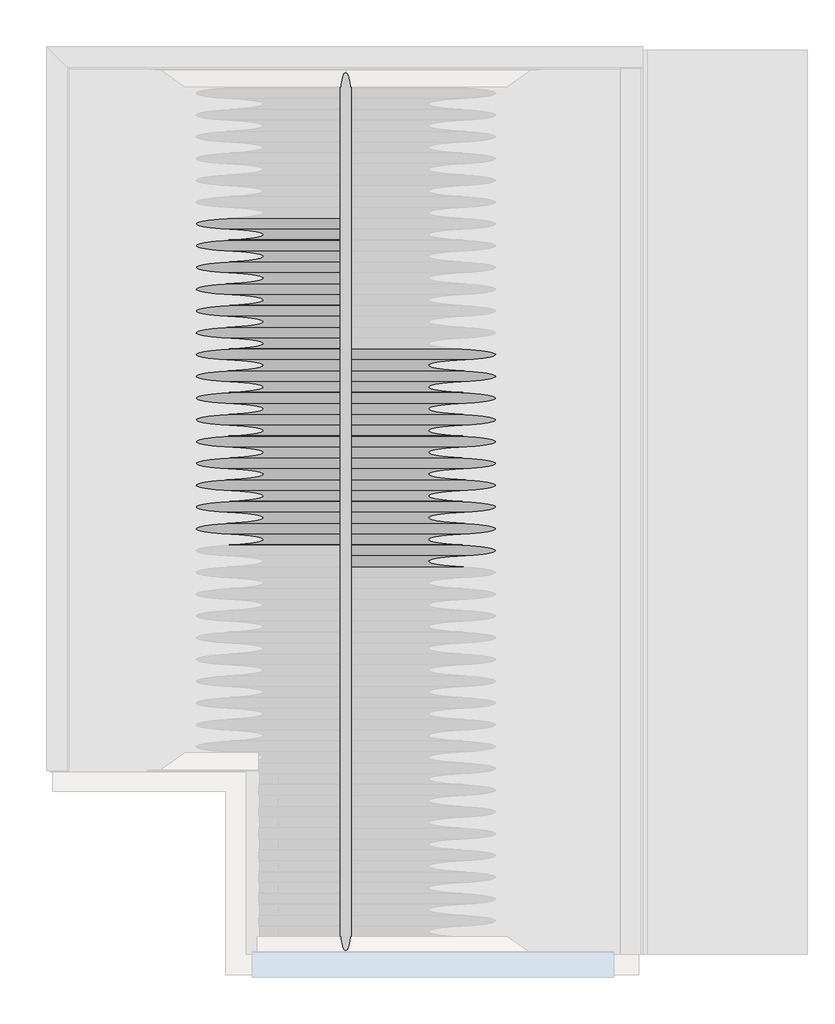
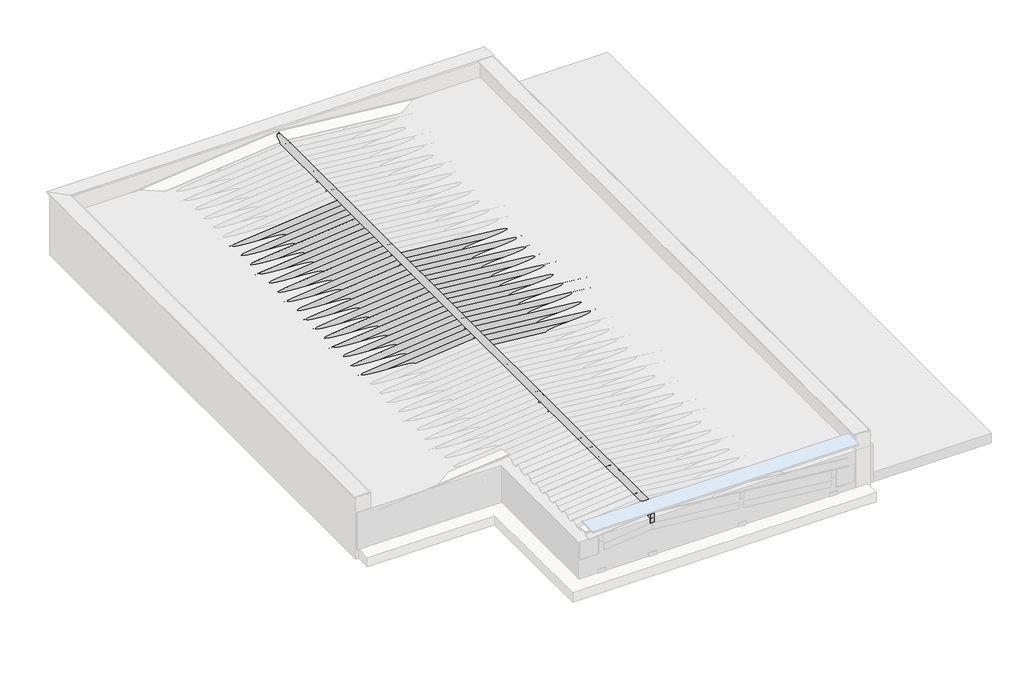
# One storey, part 3 of 4: 34 beams, 7 columns.
"""IFC4 building model written with IfcOpenShell, lengths in millimetres."""

import ifcopenshell
import ifcopenshell.guid

model = None  # the IFC model being written
_history = None  # IfcOwnerHistory: only IFC2X3 demands one
_inside = {}  # id of a spatial element -> (the spatial element, [elements in it])
_under = {}  # id of a project, library or spatial element -> (it, [spatial elements below it])
_declared = {}  # id of a project -> (the project, [libraries it declares])
_typed = {}  # id of a type object -> (the type object, [elements of that type])
_made_of = {}  # id of a material, layer set ... -> (it, [elements and type objects made of it])


def new_model(schema):
    """Start an empty IFC model of exactly this schema.

    Asked for "IFC4X3", IfcOpenShell would pick the latest addendum, in which some entities
    have other attributes; the version numbers below select the first issue.
    IFC2X3 requires an IfcOwnerHistory on every rooted entity: one is made here for all.
    """
    global model, _history
    if schema == "IFC4X3":
        model = ifcopenshell.file(schema_version=(4, 3, 0, 0))
    else:
        model = ifcopenshell.file(schema=schema)
    _inside.clear()
    _under.clear()
    _declared.clear()
    _typed.clear()
    _made_of.clear()
    _history = None
    if model.schema == "IFC2X3":
        org = make("IfcOrganization", Name="unknown")
        user = make(
            "IfcPersonAndOrganization",
            ThePerson=make("IfcPerson", FamilyName="unknown"),
            TheOrganization=org,
        )
        app = make(
            "IfcApplication",
            ApplicationDeveloper=org,
            Version="unknown",
            ApplicationFullName="unknown",
            ApplicationIdentifier="unknown",
        )
        _history = make(
            "IfcOwnerHistory",
            OwningUser=user,
            OwningApplication=app,
            ChangeAction="ADDED",
            CreationDate=0,
        )
    return model


def make(cls, **values):
    """One entity of the class cls with the attributes given. An attribute that is None is left unset."""
    return model.create_entity(
        cls, **{name: value for name, value in values.items() if value is not None}
    )


def rooted(cls, **values):
    """An entity with a GlobalId (a new one), such as an element, a storey or a relation."""
    return make(cls, GlobalId=ifcopenshell.guid.new(), OwnerHistory=_history, **values)


def si_unit(unit_type, name, prefix=None):
    """IfcSIUnit, for example si_unit("LENGTHUNIT", "METRE", prefix="MILLI")."""
    return make("IfcSIUnit", UnitType=unit_type, Prefix=prefix, Name=name)


def assignment(units):
    """IfcUnitAssignment: the units of a project."""
    return None if units is None else make("IfcUnitAssignment", Units=units)


def point(xyz):
    """IfcCartesianPoint."""
    return None if xyz is None else make("IfcCartesianPoint", Coordinates=xyz)


def direction(xyz):
    """IfcDirection."""
    return None if xyz is None else make("IfcDirection", DirectionRatios=xyz)


def frame(location, z_axis=None, x_axis=None):
    """IfcAxis2Placement3D, a coordinate frame: its origin and axes. An axis left out is left unset."""
    return make(
        "IfcAxis2Placement3D",
        Location=point(location),
        Axis=direction(z_axis),
        RefDirection=direction(x_axis),
    )


def frame_2d(location, x_axis=None):
    """IfcAxis2Placement2D, a coordinate frame in the plane: its origin and x axis."""
    return make(
        "IfcAxis2Placement2D", Location=point(location), RefDirection=direction(x_axis)
    )


def origin():
    """The frame at (0, 0, 0) with its axes left unset."""
    return frame((0.0, 0.0, 0.0))


def place(relative_to, where):
    """IfcLocalPlacement: puts the frame where relative to a parent placement (None: the world)."""
    return make(
        "IfcLocalPlacement", PlacementRelTo=relative_to, RelativePlacement=where
    )


def context(
    kind, dimensions, precision=None, world=None, true_north=None, identifier=None
):
    """IfcGeometricRepresentationContext, for example the 3D "Model" context."""
    return make(
        "IfcGeometricRepresentationContext",
        ContextIdentifier=identifier,
        ContextType=kind,
        CoordinateSpaceDimension=dimensions,
        Precision=precision,
        WorldCoordinateSystem=world,
        TrueNorth=true_north,
    )


def project(units=None, contexts=None):
    """IfcProject with its units and contexts."""
    return rooted(
        "IfcProject",
        Name="project",
        RepresentationContexts=contexts,
        UnitsInContext=assignment(units),
    )


def spatial(cls, under=None, at=None, **own):
    """A site, building, storey or space (cls), placed at a placement, below another one or the project."""
    s = rooted(cls, ObjectPlacement=at, **own)
    if under is not None:
        _under.setdefault(under.id(), (under, []))[1].append(s)
    return s


def polyline(points):
    """IfcPolyline through the points."""
    return make("IfcPolyline", Points=[point(p) for p in points])


def circle_curve(where, radius):
    """IfcCircle in the frame where."""
    return make("IfcCircle", Position=where, Radius=radius)


def trimmed(basis, trim1, trim2, sense, master):
    """IfcTrimmedCurve: the piece of a basis curve between two trims."""
    return make(
        "IfcTrimmedCurve",
        BasisCurve=basis,
        Trim1=trim1,
        Trim2=trim2,
        SenseAgreement=sense,
        MasterRepresentation=master,
    )


def segment(curve, same_sense, transition):
    """IfcCompositeCurveSegment."""
    return make(
        "IfcCompositeCurveSegment",
        Transition=transition,
        SameSense=same_sense,
        ParentCurve=curve,
    )


def composite_curve(segments, self_intersect=None):
    """IfcCompositeCurve: segments joined end to end."""
    return make("IfcCompositeCurve", Segments=segments, SelfIntersect=self_intersect)


def outline(outer, holes=None, kind="AREA"):
    """IfcArbitraryClosedProfileDef: a profile drawn as a closed curve; with holes, ...WithVoids."""
    if holes is None:
        return make("IfcArbitraryClosedProfileDef", ProfileType=kind, OuterCurve=outer)
    return make(
        "IfcArbitraryProfileDefWithVoids",
        ProfileType=kind,
        OuterCurve=outer,
        InnerCurves=holes,
    )


def extrude(swept, where, along, depth):
    """IfcExtrudedAreaSolid: the profile swept, set in the frame where, extruded along a direction by depth."""
    return make(
        "IfcExtrudedAreaSolid",
        SweptArea=swept,
        Position=where,
        ExtrudedDirection=direction(along),
        Depth=depth,
    )


def shape(context_of_items, identifier, shape_type, items):
    """IfcShapeRepresentation: the items that make up one representation, for example the "Body"."""
    return make(
        "IfcShapeRepresentation",
        ContextOfItems=context_of_items,
        RepresentationIdentifier=identifier,
        RepresentationType=shape_type,
        Items=items,
    )


def source(mapping_origin, context_of_items, identifier, shape_type, items):
    """IfcRepresentationMap: a shape defined once, which mapped items show again and again."""
    return make(
        "IfcRepresentationMap",
        MappingOrigin=mapping_origin,
        MappedRepresentation=shape(context_of_items, identifier, shape_type, items),
    )


def transform(
    local_origin,
    x_axis=None,
    y_axis=None,
    z_axis=None,
    scale=None,
    scale2=None,
    scale3=None,
    uniform=True,
):
    """IfcCartesianTransformationOperator3D, or its non-uniform kind. x_axis, y_axis, z_axis: its Axis1, 2, 3."""
    if uniform:
        return make(
            "IfcCartesianTransformationOperator3D",
            Axis1=direction(x_axis),
            Axis2=direction(y_axis),
            LocalOrigin=point(local_origin),
            Scale=scale,
            Axis3=direction(z_axis),
        )
    return make(
        "IfcCartesianTransformationOperator3DnonUniform",
        Axis1=direction(x_axis),
        Axis2=direction(y_axis),
        LocalOrigin=point(local_origin),
        Scale=scale,
        Axis3=direction(z_axis),
        Scale2=scale2,
        Scale3=scale3,
    )


def mapped(mapping_source, mapping_target):
    """IfcMappedItem: shows the shape of a source again, moved by a transform."""
    return make(
        "IfcMappedItem", MappingSource=mapping_source, MappingTarget=mapping_target
    )


def made_of(thing, what):
    """Note that an element or type object is made of a material, layer set ...; save() writes the relation."""
    if what is not None:
        _made_of.setdefault(what.id(), (what, []))[1].append(thing)
    return thing


def element(
    cls,
    number,
    at=None,
    inside=None,
    cuts=None,
    type_object=None,
    material=None,
    context=None,
    identifier="Body",
    shape_type=None,
    held_by="IfcProductDefinitionShape",
    body=None,
    shapes=None,
    **own,
):
    """One element of the class cls, such as IfcWall. Its Tag is "e" and its number.

    at: its placement. inside: the storey or other place that contains it. cuts: it is an
    opening in that element (IfcRelVoidsElement). A single representation is given by context,
    identifier, shape_type and body (its items); several are given by shapes. held_by: the class
    of the entity that holds the representations. save() writes the other relations.
    """
    e = rooted(cls, Tag="e%d" % number, ObjectPlacement=at, **own)
    if body is not None:
        shapes = [shape(context, identifier, shape_type, body)]
    if shapes is not None:
        e.Representation = make(held_by, Representations=shapes)
    if inside is not None:
        _inside.setdefault(inside.id(), (inside, []))[1].append(e)
    if cuts is not None:
        rooted(
            "IfcRelVoidsElement", RelatingBuildingElement=cuts, RelatedOpeningElement=e
        )
    if type_object is not None:
        _typed.setdefault(type_object.id(), (type_object, []))[1].append(e)
    return made_of(e, material)


def aggregate(whole, parts):
    """IfcRelAggregates: a whole, such as a stair, and the parts it consists of."""
    return rooted("IfcRelAggregates", RelatingObject=whole, RelatedObjects=parts)


def save(model, path):
    """Write the relations noted so far, then the file.

    IfcRelAggregates (storeys below a building ...), IfcRelContainedInSpatialStructure (elements
    in a storey), IfcRelDefinesByType, IfcRelAssociatesMaterial and IfcRelDeclares: one each for
    every whole, place, type object, material and project.
    """
    for whole, parts in _under.values():
        aggregate(whole, parts)
    for where, things in _inside.values():
        rooted(
            "IfcRelContainedInSpatialStructure",
            RelatedElements=things,
            RelatingStructure=where,
        )
    for kind, things in _typed.values():
        rooted("IfcRelDefinesByType", RelatedObjects=things, RelatingType=kind)
    for what, things in _made_of.values():
        rooted("IfcRelAssociatesMaterial", RelatedObjects=things, RelatingMaterial=what)
    for by, libraries in _declared.values():
        rooted("IfcRelDeclares", RelatingContext=by, RelatedDefinitions=libraries)
    model.write(path)


def cumeeira_telha_ondulada_fibrocimento_c9eafb3e(model_context):
    return source(origin(), model_context, "Body", "SweptSolid", [
        extrude(outline(composite_curve([segment(polyline([(58.3970135, 42.4437972), (53.9055884, 40.2467307)]), True, "CONTINUOUS"), segment(trimmed(circle_curve(frame_2d((-1.6029865, 13.0936483)), 61.7939461), [point((53.9055884, 40.2467307))], [point((-57.1115615, 40.2467307))], True, "CARTESIAN"), True, "CONTINUOUS"), segment(polyline([(-57.1115615, 40.2467307), (-61.6029865, 42.4437972)]), True, "CONTINUOUS"), segment(trimmed(circle_curve(frame_2d((-1.6029865, 13.0936483)), 66.7939461), [point((-61.6029865, 42.4437972))], [point((58.3970135, 42.4437972))], False, "CARTESIAN"), True, "CONTINUOUS")], self_intersect=False)), frame((-4969.5, 0.0, 0.0), z_axis=(1.0, 0.0, 0.0), x_axis=(0.0, 1.0, 0.0)), (0.0, 0.0, 1.0), 9939.0),
    ])


def viga_cumeeira_6x16cm_10b61863(model_context):
    return source(origin(), model_context, "Body", "SweptSolid", [
        extrude(outline(polyline([(4969.4999994, 30.0), (4969.4999994, -30.0), (-4969.4999994, -30.0), (-4969.4999994, 30.0), (4969.4999994, 30.0)])), frame((0.0, 0.0, -80.0), z_axis=(0.0, 0.0, 1.0), x_axis=(1.0, 0.0, 0.0)), (0.0, 0.0, 1.0), 160.0),
    ])


def column_7d6827b5(model_context):
    return source(origin(), model_context, "Body", "SweptSolid", [
        extrude(outline(polyline([(30.0, 80.0), (30.0, -80.0), (-30.0, -80.0), (-30.0, 80.0), (30.0, 80.0)])), frame((0.0, 0.0, 4460.0), z_axis=(0.0, 0.0, 1.0), x_axis=(1.0, 0.0, 0.0)), (0.0, 0.0, 1.0), 466.0),
    ])


def column_c7348c99(model_context):
    return source(origin(), model_context, "Body", "SweptSolid", [
        extrude(outline(polyline([(30.0, 80.0), (30.0, -80.0), (-30.0, -80.0), (-30.0, 80.0), (30.0, 80.0)])), frame((0.0, 0.0, 4460.0), z_axis=(0.0, 0.0, 1.0), x_axis=(1.0, 0.0, 0.0)), (0.0, 0.0, 1.0), 372.8),
    ])


def column_6cc9e01b(model_context):
    return source(origin(), model_context, "Body", "SweptSolid", [
        extrude(outline(polyline([(30.0, 80.0), (30.0, -80.0), (-30.0, -80.0), (-30.0, 80.0), (30.0, 80.0)])), frame((0.0, 0.0, 4460.0), z_axis=(0.0, 0.0, 1.0), x_axis=(1.0, 0.0, 0.0)), (0.0, 0.0, 1.0), 233.0),
    ])


model = new_model("IFC4")

# Units and contexts
model_context = context("Model", 3, world=origin())
ifc_project = project(units=[si_unit("LENGTHUNIT", "METRE", prefix="MILLI")], contexts=[model_context])

# Site, building, storey
site = spatial("IfcSite", under=ifc_project)
building = spatial("IfcBuilding", under=site)
storey = spatial("IfcBuildingStorey", under=building, Name="COB. SALA ESTAR", Elevation=4400.0)

# Beams
placement = place(None, origin())
element("IfcBeam", 1, ObjectType="Madeira de lei : Berço 6x12cm", at=placement, inside=storey, context=model_context, shape_type="SweptSolid", body=[
    extrude(outline(polyline([(-3400.8557491, 2180.4300147), (-3280.8557491, 2180.4300147), (-3280.8557491, 180.4300153), (-3400.8557491, 180.4300153), (-3400.8557491, 2180.4300147)])), frame((0.0, 0.0, 4400.0), z_axis=(0.0, 0.0, 1.0), x_axis=(1.0, 0.0, 0.0)), (0.0, 0.0, 1.0), 60.0),
])
element("IfcBeam", 2, ObjectType="Madeira de lei : Berço 6x12cm", at=placement, inside=storey, context=model_context, shape_type="SweptSolid", body=[
    extrude(outline(polyline([(-3400.8557491, 4180.4300153), (-3280.8557491, 4180.4300153), (-3280.8557491, 2180.4300159), (-3400.8557491, 2180.4300159), (-3400.8557491, 4180.4300153)])), frame((0.0, 0.0, 4400.0), z_axis=(0.0, 0.0, 1.0), x_axis=(1.0, 0.0, 0.0)), (0.0, 0.0, 1.0), 60.0),
])
element("IfcBeam", 3, ObjectType="Madeira de lei : Berço 6x12cm", at=placement, inside=storey, context=model_context, shape_type="SweptSolid", body=[
    extrude(outline(polyline([(-2032.3324227, 2180.4300147), (-1912.3324227, 2180.4300147), (-1912.3324227, 180.4300153), (-2032.3324227, 180.4300153), (-2032.3324227, 2180.4300147)])), frame((0.0, 0.0, 4400.0), z_axis=(0.0, 0.0, 1.0), x_axis=(1.0, 0.0, 0.0)), (0.0, 0.0, 1.0), 60.0),
])
element("IfcBeam", 4, ObjectType="Madeira de lei : Berço 6x12cm", at=placement, inside=storey, context=model_context, shape_type="SweptSolid", body=[
    extrude(outline(polyline([(-634.0324227, 2180.4300147), (-514.0324227, 2180.4300147), (-514.0324227, 180.4300153), (-634.0324227, 180.4300153), (-634.0324227, 2180.4300147)])), frame((0.0, 0.0, 4400.0), z_axis=(0.0, 0.0, 1.0), x_axis=(1.0, 0.0, 0.0)), (0.0, 0.0, 1.0), 60.0),
])
element("IfcBeam", 5, ObjectType="Madeira de lei : Berço 6x12cm", at=placement, inside=storey, context=model_context, shape_type="SweptSolid", body=[
    extrude(outline(polyline([(-6167.5301913, 4180.4300153), (-6047.5301913, 4180.4300153), (-6047.5301913, 2180.4300159), (-6167.5301913, 2180.4300159), (-6167.5301913, 4180.4300153)])), frame((0.0, 0.0, 4400.0), z_axis=(0.0, 0.0, 1.0), x_axis=(1.0, 0.0, 0.0)), (0.0, 0.0, 1.0), 60.0),
])
element("IfcBeam", 6, ObjectType="Madeira de lei : Berço 6x12cm", at=placement, inside=storey, context=model_context, shape_type="SweptSolid", body=[
    extrude(outline(polyline([(-4769.2301913, 2180.4300147), (-4649.2301913, 2180.4300147), (-4649.2301913, 180.4300153), (-4769.2301913, 180.4300153), (-4769.2301913, 2180.4300147)])), frame((0.0, 0.0, 4400.0), z_axis=(0.0, 0.0, 1.0), x_axis=(1.0, 0.0, 0.0)), (0.0, 0.0, 1.0), 60.0),
])
element("IfcBeam", 7, ObjectType="Madeira de lei : Berço 6x12cm", at=placement, inside=storey, context=model_context, shape_type="SweptSolid", body=[
    extrude(outline(polyline([(-4769.2301913, 4180.4300153), (-4649.2301913, 4180.4300153), (-4649.2301913, 2180.4300159), (-4769.2301913, 2180.4300159), (-4769.2301913, 4180.4300153)])), frame((0.0, 0.0, 4400.0), z_axis=(0.0, 0.0, 1.0), x_axis=(1.0, 0.0, 0.0)), (0.0, 0.0, 1.0), 60.0),
])
cumeeira_telha_ondulada_fibrocimento_shape = cumeeira_telha_ondulada_fibrocimento_c9eafb3e(model_context)
element("IfcBeam", 8, ObjectType="Cumeeira Telha Ondulada : Fibrocimento", at=placement, inside=storey, context=model_context, shape_type="MappedRepresentation", body=[
    mapped(cumeeira_telha_ondulada_fibrocimento_shape, transform((-3340.8557491, 623.9300153, 5123.1251229), x_axis=(0.0, -1.0, 0.0), y_axis=(1.0, 0.0, 0.0), z_axis=(0.0, 0.0, 1.0))),
])
element("IfcBeam", 9, ObjectType="Telha Ondulada : Fibrocimento", at=placement, inside=storey, context=model_context, shape_type="SweptSolid", body=[
    extrude(outline(composite_curve([segment(trimmed(circle_curve(frame_2d((-58.7002978, -53.2060538)), 66.7939461), [point((-29.3501489, 6.7939462))], [point((-29.3501489, -113.2060538))], False, "CARTESIAN"), True, "CONTINUOUS"), segment(polyline([(-29.3501489, -113.2060538), (-31.5472154, -108.7146288)]), True, "CONTINUOUS"), segment(trimmed(circle_curve(frame_2d((-58.7002978, -53.2060538)), 61.7939461), [point((-31.5472154, -108.7146288))], [point((-31.5472154, 2.3025211))], True, "CARTESIAN"), True, "CONTINUOUS"), segment(trimmed(circle_curve(frame_2d((0.0, 66.7939462)), 71.7939461), [point((-31.5472154, 2.3025211))], [point((-31.5472154, 131.2853712))], False, "CARTESIAN"), True, "CONTINUOUS"), segment(polyline([(-31.5472154, 131.2853712), (-29.3501489, 126.7939462)]), True, "CONTINUOUS"), segment(trimmed(circle_curve(frame_2d((0.0, 66.7939462)), 66.7939461), [point((-29.3501489, 126.7939462))], [point((-29.3501489, 6.7939462))], True, "CARTESIAN"), True, "CONTINUOUS")], self_intersect=False)), frame((-6307.6707245, 377.826948, 4862.7215886), z_axis=(0.9950371902099892, 0.0, 0.09950371902099972), x_axis=(-0.09950371902099972, 0.0, 0.9950371902099892)), (0.0, 0.0, 1.0), 2972.5075682),
])
element("IfcBeam", 10, ObjectType="Telha Ondulada : Fibrocimento", at=placement, inside=storey, context=model_context, shape_type="SweptSolid", body=[
    extrude(outline(composite_curve([segment(trimmed(circle_curve(frame_2d((-58.7002978, -53.2060538)), 66.7939461), [point((-29.3501489, 6.7939462))], [point((-29.3501489, -113.2060538))], False, "CARTESIAN"), True, "CONTINUOUS"), segment(polyline([(-29.3501489, -113.2060538), (-31.5472154, -108.7146288)]), True, "CONTINUOUS"), segment(trimmed(circle_curve(frame_2d((-58.7002978, -53.2060538)), 61.7939461), [point((-31.5472154, -108.7146288))], [point((-31.5472154, 2.3025211))], True, "CARTESIAN"), True, "CONTINUOUS"), segment(trimmed(circle_curve(frame_2d((0.0, 66.7939462)), 71.7939461), [point((-31.5472154, 2.3025211))], [point((-31.5472154, 131.2853712))], False, "CARTESIAN"), True, "CONTINUOUS"), segment(polyline([(-31.5472154, 131.2853712), (-29.3501489, 126.7939462)]), True, "CONTINUOUS"), segment(trimmed(circle_curve(frame_2d((0.0, 66.7939462)), 66.7939461), [point((-29.3501489, 126.7939462))], [point((-29.3501489, 6.7939462))], True, "CARTESIAN"), True, "CONTINUOUS")], self_intersect=False)), frame((-6307.6707245, 622.326948, 4862.7215886), z_axis=(0.9950371902099892, 0.0, 0.09950371902099972), x_axis=(-0.09950371902099972, 0.0, 0.9950371902099892)), (0.0, 0.0, 1.0), 2972.5075682),
])
element("IfcBeam", 11, ObjectType="Telha Ondulada : Fibrocimento", at=placement, inside=storey, context=model_context, shape_type="SweptSolid", body=[
    extrude(outline(composite_curve([segment(trimmed(circle_curve(frame_2d((-58.7002978, -53.2060538)), 66.7939461), [point((-29.3501489, 6.7939462))], [point((-29.3501489, -113.2060538))], False, "CARTESIAN"), True, "CONTINUOUS"), segment(polyline([(-29.3501489, -113.2060538), (-31.5472154, -108.7146288)]), True, "CONTINUOUS"), segment(trimmed(circle_curve(frame_2d((-58.7002978, -53.2060538)), 61.7939461), [point((-31.5472154, -108.7146288))], [point((-31.5472154, 2.3025211))], True, "CARTESIAN"), True, "CONTINUOUS"), segment(trimmed(circle_curve(frame_2d((0.0, 66.7939462)), 71.7939461), [point((-31.5472154, 2.3025211))], [point((-31.5472154, 131.2853712))], False, "CARTESIAN"), True, "CONTINUOUS"), segment(polyline([(-31.5472154, 131.2853712), (-29.3501489, 126.7939462)]), True, "CONTINUOUS"), segment(trimmed(circle_curve(frame_2d((0.0, 66.7939462)), 66.7939461), [point((-29.3501489, 126.7939462))], [point((-29.3501489, 6.7939462))], True, "CARTESIAN"), True, "CONTINUOUS")], self_intersect=False)), frame((-6307.6707245, 866.826948, 4862.7215886), z_axis=(0.9950371902099892, 0.0, 0.09950371902099968), x_axis=(-0.09950371902099968, 0.0, 0.9950371902099892)), (0.0, 0.0, 1.0), 2972.5075682),
])
element("IfcBeam", 12, ObjectType="Telha Ondulada : Fibrocimento", at=placement, inside=storey, context=model_context, shape_type="SweptSolid", body=[
    extrude(outline(composite_curve([segment(trimmed(circle_curve(frame_2d((-58.7002978, -53.2060538)), 66.7939461), [point((-29.3501489, 6.7939462))], [point((-29.3501489, -113.2060538))], False, "CARTESIAN"), True, "CONTINUOUS"), segment(polyline([(-29.3501489, -113.2060538), (-31.5472154, -108.7146288)]), True, "CONTINUOUS"), segment(trimmed(circle_curve(frame_2d((-58.7002978, -53.2060538)), 61.7939461), [point((-31.5472154, -108.7146288))], [point((-31.5472154, 2.3025211))], True, "CARTESIAN"), True, "CONTINUOUS"), segment(trimmed(circle_curve(frame_2d((0.0, 66.7939462)), 71.7939461), [point((-31.5472154, 2.3025211))], [point((-31.5472154, 131.2853712))], False, "CARTESIAN"), True, "CONTINUOUS"), segment(polyline([(-31.5472154, 131.2853712), (-29.3501489, 126.7939462)]), True, "CONTINUOUS"), segment(trimmed(circle_curve(frame_2d((0.0, 66.7939462)), 66.7939461), [point((-29.3501489, 126.7939462))], [point((-29.3501489, 6.7939462))], True, "CARTESIAN"), True, "CONTINUOUS")], self_intersect=False)), frame((-6307.6707245, 1111.326948, 4862.7215886), z_axis=(0.9950371902099892, 0.0, 0.09950371902099972), x_axis=(-0.09950371902099972, 0.0, 0.9950371902099892)), (0.0, 0.0, 1.0), 2972.5075682),
])
element("IfcBeam", 13, ObjectType="Telha Ondulada : Fibrocimento", at=placement, inside=storey, context=model_context, shape_type="SweptSolid", body=[
    extrude(outline(composite_curve([segment(trimmed(circle_curve(frame_2d((-58.7002978, -53.2060538)), 66.7939461), [point((-29.3501489, 6.7939462))], [point((-29.3501489, -113.2060538))], False, "CARTESIAN"), True, "CONTINUOUS"), segment(polyline([(-29.3501489, -113.2060538), (-31.5472154, -108.7146288)]), True, "CONTINUOUS"), segment(trimmed(circle_curve(frame_2d((-58.7002978, -53.2060538)), 61.7939461), [point((-31.5472154, -108.7146288))], [point((-31.5472154, 2.3025211))], True, "CARTESIAN"), True, "CONTINUOUS"), segment(trimmed(circle_curve(frame_2d((0.0, 66.7939462)), 71.7939461), [point((-31.5472154, 2.3025211))], [point((-31.5472154, 131.2853712))], False, "CARTESIAN"), True, "CONTINUOUS"), segment(polyline([(-31.5472154, 131.2853712), (-29.3501489, 126.7939462)]), True, "CONTINUOUS"), segment(trimmed(circle_curve(frame_2d((0.0, 66.7939462)), 66.7939461), [point((-29.3501489, 126.7939462))], [point((-29.3501489, 6.7939462))], True, "CARTESIAN"), True, "CONTINUOUS")], self_intersect=False)), frame((-6307.6707245, 1355.826948, 4862.7215886), z_axis=(0.9950371902099892, 0.0, 0.09950371902099969), x_axis=(-0.09950371902099969, 0.0, 0.9950371902099892)), (0.0, 0.0, 1.0), 2972.5075682),
])
element("IfcBeam", 14, ObjectType="Telha Ondulada : Fibrocimento", at=placement, inside=storey, context=model_context, shape_type="SweptSolid", body=[
    extrude(outline(composite_curve([segment(trimmed(circle_curve(frame_2d((-58.7002978, -53.2060538)), 66.7939461), [point((-29.3501489, 6.7939462))], [point((-29.3501489, -113.2060538))], False, "CARTESIAN"), True, "CONTINUOUS"), segment(polyline([(-29.3501489, -113.2060538), (-31.5472154, -108.7146288)]), True, "CONTINUOUS"), segment(trimmed(circle_curve(frame_2d((-58.7002978, -53.2060538)), 61.7939461), [point((-31.5472154, -108.7146288))], [point((-31.5472154, 2.3025211))], True, "CARTESIAN"), True, "CONTINUOUS"), segment(trimmed(circle_curve(frame_2d((0.0, 66.7939462)), 71.7939461), [point((-31.5472154, 2.3025211))], [point((-31.5472154, 131.2853712))], False, "CARTESIAN"), True, "CONTINUOUS"), segment(polyline([(-31.5472154, 131.2853712), (-29.3501489, 126.7939462)]), True, "CONTINUOUS"), segment(trimmed(circle_curve(frame_2d((0.0, 66.7939462)), 66.7939461), [point((-29.3501489, 126.7939462))], [point((-29.3501489, 6.7939462))], True, "CARTESIAN"), True, "CONTINUOUS")], self_intersect=False)), frame((-6307.6707245, 1600.326948, 4862.7215886), z_axis=(0.9950371902099892, 0.0, 0.09950371902099972), x_axis=(-0.09950371902099972, 0.0, 0.9950371902099892)), (0.0, 0.0, 1.0), 2972.5075682),
])
element("IfcBeam", 15, ObjectType="Telha Ondulada : Fibrocimento", at=placement, inside=storey, context=model_context, shape_type="SweptSolid", body=[
    extrude(outline(composite_curve([segment(trimmed(circle_curve(frame_2d((-58.7002978, -53.2060538)), 66.7939461), [point((-29.3501489, 6.7939462))], [point((-29.3501489, -113.2060538))], False, "CARTESIAN"), True, "CONTINUOUS"), segment(polyline([(-29.3501489, -113.2060538), (-31.5472154, -108.7146288)]), True, "CONTINUOUS"), segment(trimmed(circle_curve(frame_2d((-58.7002978, -53.2060538)), 61.7939461), [point((-31.5472154, -108.7146288))], [point((-31.5472154, 2.3025211))], True, "CARTESIAN"), True, "CONTINUOUS"), segment(trimmed(circle_curve(frame_2d((0.0, 66.7939462)), 71.7939461), [point((-31.5472154, 2.3025211))], [point((-31.5472154, 131.2853712))], False, "CARTESIAN"), True, "CONTINUOUS"), segment(polyline([(-31.5472154, 131.2853712), (-29.3501489, 126.7939462)]), True, "CONTINUOUS"), segment(trimmed(circle_curve(frame_2d((0.0, 66.7939462)), 66.7939461), [point((-29.3501489, 126.7939462))], [point((-29.3501489, 6.7939462))], True, "CARTESIAN"), True, "CONTINUOUS")], self_intersect=False)), frame((-6307.6707245, 1844.826948, 4862.7215886), z_axis=(0.9950371902099892, 0.0, 0.09950371902099972), x_axis=(-0.09950371902099972, 0.0, 0.9950371902099892)), (0.0, 0.0, 1.0), 2972.5075682),
])
element("IfcBeam", 16, ObjectType="Telha Ondulada : Fibrocimento", at=placement, inside=storey, context=model_context, shape_type="SweptSolid", body=[
    extrude(outline(composite_curve([segment(trimmed(circle_curve(frame_2d((-58.7002978, -53.2060538)), 66.7939461), [point((-29.3501489, 6.7939462))], [point((-29.3501489, -113.2060538))], False, "CARTESIAN"), True, "CONTINUOUS"), segment(polyline([(-29.3501489, -113.2060538), (-31.5472154, -108.7146288)]), True, "CONTINUOUS"), segment(trimmed(circle_curve(frame_2d((-58.7002978, -53.2060538)), 61.7939461), [point((-31.5472154, -108.7146288))], [point((-31.5472154, 2.3025211))], True, "CARTESIAN"), True, "CONTINUOUS"), segment(trimmed(circle_curve(frame_2d((0.0, 66.7939462)), 71.7939461), [point((-31.5472154, 2.3025211))], [point((-31.5472154, 131.2853712))], False, "CARTESIAN"), True, "CONTINUOUS"), segment(polyline([(-31.5472154, 131.2853712), (-29.3501489, 126.7939462)]), True, "CONTINUOUS"), segment(trimmed(circle_curve(frame_2d((0.0, 66.7939462)), 66.7939461), [point((-29.3501489, 126.7939462))], [point((-29.3501489, 6.7939462))], True, "CARTESIAN"), True, "CONTINUOUS")], self_intersect=False)), frame((-6307.6707245, 2089.326948, 4862.7215886), z_axis=(0.9950371902099892, 0.0, 0.09950371902099954), x_axis=(-0.09950371902099954, 0.0, 0.9950371902099892)), (0.0, 0.0, 1.0), 2972.5075682),
])
element("IfcBeam", 17, ObjectType="Telha Ondulada : Fibrocimento", at=placement, inside=storey, context=model_context, shape_type="SweptSolid", body=[
    extrude(outline(composite_curve([segment(trimmed(circle_curve(frame_2d((-58.7002978, -53.2060538)), 66.7939461), [point((-29.3501489, 6.7939462))], [point((-29.3501489, -113.2060538))], False, "CARTESIAN"), True, "CONTINUOUS"), segment(polyline([(-29.3501489, -113.2060538), (-31.5472154, -108.7146288)]), True, "CONTINUOUS"), segment(trimmed(circle_curve(frame_2d((-58.7002978, -53.2060538)), 61.7939461), [point((-31.5472154, -108.7146288))], [point((-31.5472154, 2.3025211))], True, "CARTESIAN"), True, "CONTINUOUS"), segment(trimmed(circle_curve(frame_2d((0.0, 66.7939462)), 71.7939461), [point((-31.5472154, 2.3025211))], [point((-31.5472154, 131.2853712))], False, "CARTESIAN"), True, "CONTINUOUS"), segment(polyline([(-31.5472154, 131.2853712), (-29.3501489, 126.7939462)]), True, "CONTINUOUS"), segment(trimmed(circle_curve(frame_2d((0.0, 66.7939462)), 66.7939461), [point((-29.3501489, 126.7939462))], [point((-29.3501489, 6.7939462))], True, "CARTESIAN"), True, "CONTINUOUS")], self_intersect=False)), frame((-6307.6707245, 2333.826948, 4862.7215886), z_axis=(0.9950371902099892, 0.0, 0.09950371902099972), x_axis=(-0.09950371902099972, 0.0, 0.9950371902099892)), (0.0, 0.0, 1.0), 2972.5075682),
])
element("IfcBeam", 18, ObjectType="Telha Ondulada : Fibrocimento", at=placement, inside=storey, context=model_context, shape_type="SweptSolid", body=[
    extrude(outline(composite_curve([segment(trimmed(circle_curve(frame_2d((-58.7002978, -53.2060538)), 66.7939461), [point((-29.3501489, 6.7939462))], [point((-29.3501489, -113.2060538))], False, "CARTESIAN"), True, "CONTINUOUS"), segment(polyline([(-29.3501489, -113.2060538), (-31.5472154, -108.7146288)]), True, "CONTINUOUS"), segment(trimmed(circle_curve(frame_2d((-58.7002978, -53.2060538)), 61.7939461), [point((-31.5472154, -108.7146288))], [point((-31.5472154, 2.3025211))], True, "CARTESIAN"), True, "CONTINUOUS"), segment(trimmed(circle_curve(frame_2d((0.0, 66.7939462)), 71.7939461), [point((-31.5472154, 2.3025211))], [point((-31.5472154, 131.2853712))], False, "CARTESIAN"), True, "CONTINUOUS"), segment(polyline([(-31.5472154, 131.2853712), (-29.3501489, 126.7939462)]), True, "CONTINUOUS"), segment(trimmed(circle_curve(frame_2d((0.0, 66.7939462)), 66.7939461), [point((-29.3501489, 126.7939462))], [point((-29.3501489, 6.7939462))], True, "CARTESIAN"), True, "CONTINUOUS")], self_intersect=False)), frame((-6307.6707245, 2578.326948, 4862.7215886), z_axis=(0.9950371902099892, 0.0, 0.09950371902099969), x_axis=(-0.09950371902099969, 0.0, 0.9950371902099892)), (0.0, 0.0, 1.0), 2972.5075682),
])
element("IfcBeam", 19, ObjectType="Telha Ondulada : Fibrocimento", at=placement, inside=storey, context=model_context, shape_type="SweptSolid", body=[
    extrude(outline(composite_curve([segment(trimmed(circle_curve(frame_2d((-58.7002978, -53.2060538)), 66.7939461), [point((-29.3501489, 6.7939462))], [point((-29.3501489, -113.2060538))], False, "CARTESIAN"), True, "CONTINUOUS"), segment(polyline([(-29.3501489, -113.2060538), (-31.5472154, -108.7146288)]), True, "CONTINUOUS"), segment(trimmed(circle_curve(frame_2d((-58.7002978, -53.2060538)), 61.7939461), [point((-31.5472154, -108.7146288))], [point((-31.5472154, 2.3025211))], True, "CARTESIAN"), True, "CONTINUOUS"), segment(trimmed(circle_curve(frame_2d((0.0, 66.7939462)), 71.7939461), [point((-31.5472154, 2.3025211))], [point((-31.5472154, 131.2853712))], False, "CARTESIAN"), True, "CONTINUOUS"), segment(polyline([(-31.5472154, 131.2853712), (-29.3501489, 126.7939462)]), True, "CONTINUOUS"), segment(trimmed(circle_curve(frame_2d((0.0, 66.7939462)), 66.7939461), [point((-29.3501489, 126.7939462))], [point((-29.3501489, 6.7939462))], True, "CARTESIAN"), True, "CONTINUOUS")], self_intersect=False)), frame((-6307.6707245, 2822.826948, 4862.7215886), z_axis=(0.9950371902099892, 0.0, 0.09950371902099972), x_axis=(-0.09950371902099972, 0.0, 0.9950371902099892)), (0.0, 0.0, 1.0), 2972.5075682),
])
element("IfcBeam", 20, ObjectType="Telha Ondulada : Fibrocimento", at=placement, inside=storey, context=model_context, shape_type="SweptSolid", body=[
    extrude(outline(composite_curve([segment(trimmed(circle_curve(frame_2d((-58.7002978, -53.2060538)), 66.7939461), [point((-29.3501489, 6.7939462))], [point((-29.3501489, -113.2060538))], False, "CARTESIAN"), True, "CONTINUOUS"), segment(polyline([(-29.3501489, -113.2060538), (-31.5472154, -108.7146288)]), True, "CONTINUOUS"), segment(trimmed(circle_curve(frame_2d((-58.7002978, -53.2060538)), 61.7939461), [point((-31.5472154, -108.7146288))], [point((-31.5472154, 2.3025211))], True, "CARTESIAN"), True, "CONTINUOUS"), segment(trimmed(circle_curve(frame_2d((0.0, 66.7939462)), 71.7939461), [point((-31.5472154, 2.3025211))], [point((-31.5472154, 131.2853712))], False, "CARTESIAN"), True, "CONTINUOUS"), segment(polyline([(-31.5472154, 131.2853712), (-29.3501489, 126.7939462)]), True, "CONTINUOUS"), segment(trimmed(circle_curve(frame_2d((0.0, 66.7939462)), 66.7939461), [point((-29.3501489, 126.7939462))], [point((-29.3501489, 6.7939462))], True, "CARTESIAN"), True, "CONTINUOUS")], self_intersect=False)), frame((-6307.6707245, 3067.326948, 4862.7215886), z_axis=(0.9950371902099892, 0.0, 0.09950371902099972), x_axis=(-0.09950371902099972, 0.0, 0.9950371902099892)), (0.0, 0.0, 1.0), 2972.5075682),
])
element("IfcBeam", 21, ObjectType="Telha Ondulada : Fibrocimento", at=placement, inside=storey, context=model_context, shape_type="SweptSolid", body=[
    extrude(outline(composite_curve([segment(trimmed(circle_curve(frame_2d((-58.7002978, -53.2060538)), 66.7939461), [point((-29.3501489, 6.7939462))], [point((-29.3501489, -113.2060538))], False, "CARTESIAN"), True, "CONTINUOUS"), segment(polyline([(-29.3501489, -113.2060538), (-31.5472154, -108.7146288)]), True, "CONTINUOUS"), segment(trimmed(circle_curve(frame_2d((-58.7002978, -53.2060538)), 61.7939461), [point((-31.5472154, -108.7146288))], [point((-31.5472154, 2.3025211))], True, "CARTESIAN"), True, "CONTINUOUS"), segment(trimmed(circle_curve(frame_2d((0.0, 66.7939462)), 71.7939461), [point((-31.5472154, 2.3025211))], [point((-31.5472154, 131.2853712))], False, "CARTESIAN"), True, "CONTINUOUS"), segment(polyline([(-31.5472154, 131.2853712), (-29.3501489, 126.7939462)]), True, "CONTINUOUS"), segment(trimmed(circle_curve(frame_2d((0.0, 66.7939462)), 66.7939461), [point((-29.3501489, 126.7939462))], [point((-29.3501489, 6.7939462))], True, "CARTESIAN"), True, "CONTINUOUS")], self_intersect=False)), frame((-6307.6707245, 3311.826948, 4862.7215886), z_axis=(0.9950371902099892, 0.0, 0.09950371902099954), x_axis=(-0.09950371902099954, 0.0, 0.9950371902099892)), (0.0, 0.0, 1.0), 2972.5075682),
])
element("IfcBeam", 22, ObjectType="Telha Ondulada : Fibrocimento", at=placement, inside=storey, context=model_context, shape_type="SweptSolid", body=[
    extrude(outline(composite_curve([segment(trimmed(circle_curve(frame_2d((-58.7002978, -53.2060538)), 66.7939461), [point((-29.3501489, 6.7939462))], [point((-29.3501489, -113.2060538))], False, "CARTESIAN"), True, "CONTINUOUS"), segment(polyline([(-29.3501489, -113.2060538), (-31.5472154, -108.7146288)]), True, "CONTINUOUS"), segment(trimmed(circle_curve(frame_2d((-58.7002978, -53.2060538)), 61.7939461), [point((-31.5472154, -108.7146288))], [point((-31.5472154, 2.3025211))], True, "CARTESIAN"), True, "CONTINUOUS"), segment(trimmed(circle_curve(frame_2d((0.0, 66.7939462)), 71.7939461), [point((-31.5472154, 2.3025211))], [point((-31.5472154, 131.2853712))], False, "CARTESIAN"), True, "CONTINUOUS"), segment(polyline([(-31.5472154, 131.2853712), (-29.3501489, 126.7939462)]), True, "CONTINUOUS"), segment(trimmed(circle_curve(frame_2d((0.0, 66.7939462)), 66.7939461), [point((-29.3501489, 126.7939462))], [point((-29.3501489, 6.7939462))], True, "CARTESIAN"), True, "CONTINUOUS")], self_intersect=False)), frame((-6307.6707245, 3556.326948, 4862.7215886), z_axis=(0.9950371902099892, 0.0, 0.09950371902099954), x_axis=(-0.09950371902099954, 0.0, 0.9950371902099892)), (0.0, 0.0, 1.0), 2972.5075682),
])
element("IfcBeam", 23, ObjectType="Telha Ondulada : Fibrocimento", at=placement, inside=storey, context=model_context, shape_type="SweptSolid", body=[
    extrude(outline(composite_curve([segment(trimmed(circle_curve(frame_2d((-58.7002978, -53.2060538)), 66.7939461), [point((-29.3501489, 6.7939462))], [point((-29.3501489, -113.2060538))], False, "CARTESIAN"), True, "CONTINUOUS"), segment(polyline([(-29.3501489, -113.2060538), (-31.5472154, -108.7146288)]), True, "CONTINUOUS"), segment(trimmed(circle_curve(frame_2d((-58.7002978, -53.2060538)), 61.7939461), [point((-31.5472154, -108.7146288))], [point((-31.5472154, 2.3025211))], True, "CARTESIAN"), True, "CONTINUOUS"), segment(trimmed(circle_curve(frame_2d((0.0, 66.7939462)), 71.7939461), [point((-31.5472154, 2.3025211))], [point((-31.5472154, 131.2853712))], False, "CARTESIAN"), True, "CONTINUOUS"), segment(polyline([(-31.5472154, 131.2853712), (-29.3501489, 126.7939462)]), True, "CONTINUOUS"), segment(trimmed(circle_curve(frame_2d((0.0, 66.7939462)), 66.7939461), [point((-29.3501489, 126.7939462))], [point((-29.3501489, 6.7939462))], True, "CARTESIAN"), True, "CONTINUOUS")], self_intersect=False)), frame((-6307.6707245, 3800.826948, 4862.7215886), z_axis=(0.9950371902099892, 0.0, 0.09950371902099968), x_axis=(-0.09950371902099968, 0.0, 0.9950371902099892)), (0.0, 0.0, 1.0), 2972.5075682),
])
element("IfcBeam", 24, ObjectType="Telha Ondulada : Fibrocimento", at=placement, inside=storey, context=model_context, shape_type="SweptSolid", body=[
    extrude(outline(composite_curve([segment(trimmed(circle_curve(frame_2d((0.0, 66.7939462)), 66.7939461), [point((29.3501489, 6.7939462))], [point((29.3501489, 126.7939462))], True, "CARTESIAN"), True, "CONTINUOUS"), segment(polyline([(29.3501489, 126.7939462), (31.5472154, 131.2853712)]), True, "CONTINUOUS"), segment(trimmed(circle_curve(frame_2d((0.0, 66.7939462)), 71.7939461), [point((31.5472154, 131.2853712))], [point((31.5472154, 2.3025211))], False, "CARTESIAN"), True, "CONTINUOUS"), segment(trimmed(circle_curve(frame_2d((58.7002978, -53.2060538)), 61.7939461), [point((31.5472154, 2.3025211))], [point((31.5472154, -108.7146288))], True, "CARTESIAN"), True, "CONTINUOUS"), segment(polyline([(31.5472154, -108.7146288), (29.3501489, -113.2060538)]), True, "CONTINUOUS"), segment(trimmed(circle_curve(frame_2d((58.7002978, -53.2060538)), 66.7939461), [point((29.3501489, -113.2060538))], [point((29.3501489, 6.7939462))], False, "CARTESIAN"), True, "CONTINUOUS")], self_intersect=False)), frame((-373.8918894, 133.326948, 4862.7215886), z_axis=(-0.9950371902099892, 0.0, 0.09950371902099946), x_axis=(-0.09950371902099946, 0.0, -0.9950371902099892)), (0.0, 0.0, 1.0), 2972.5075682),
])
element("IfcBeam", 25, ObjectType="Telha Ondulada : Fibrocimento", at=placement, inside=storey, context=model_context, shape_type="SweptSolid", body=[
    extrude(outline(composite_curve([segment(trimmed(circle_curve(frame_2d((0.0, 66.7939462)), 66.7939461), [point((29.3501489, 6.7939462))], [point((29.3501489, 126.7939462))], True, "CARTESIAN"), True, "CONTINUOUS"), segment(polyline([(29.3501489, 126.7939462), (31.5472154, 131.2853712)]), True, "CONTINUOUS"), segment(trimmed(circle_curve(frame_2d((0.0, 66.7939462)), 71.7939461), [point((31.5472154, 131.2853712))], [point((31.5472154, 2.3025211))], False, "CARTESIAN"), True, "CONTINUOUS"), segment(trimmed(circle_curve(frame_2d((58.7002978, -53.2060538)), 61.7939461), [point((31.5472154, 2.3025211))], [point((31.5472154, -108.7146288))], True, "CARTESIAN"), True, "CONTINUOUS"), segment(polyline([(31.5472154, -108.7146288), (29.3501489, -113.2060538)]), True, "CONTINUOUS"), segment(trimmed(circle_curve(frame_2d((58.7002978, -53.2060538)), 66.7939461), [point((29.3501489, -113.2060538))], [point((29.3501489, 6.7939462))], False, "CARTESIAN"), True, "CONTINUOUS")], self_intersect=False)), frame((-373.8918894, 377.826948, 4862.7215886), z_axis=(-0.9950371902099892, 0.0, 0.09950371902099946), x_axis=(-0.09950371902099946, 0.0, -0.9950371902099892)), (0.0, 0.0, 1.0), 2972.5075682),
])
element("IfcBeam", 26, ObjectType="Telha Ondulada : Fibrocimento", at=placement, inside=storey, context=model_context, shape_type="SweptSolid", body=[
    extrude(outline(composite_curve([segment(trimmed(circle_curve(frame_2d((0.0, 66.7939462)), 66.7939461), [point((29.3501489, 6.7939462))], [point((29.3501489, 126.7939462))], True, "CARTESIAN"), True, "CONTINUOUS"), segment(polyline([(29.3501489, 126.7939462), (31.5472154, 131.2853712)]), True, "CONTINUOUS"), segment(trimmed(circle_curve(frame_2d((0.0, 66.7939462)), 71.7939461), [point((31.5472154, 131.2853712))], [point((31.5472154, 2.3025211))], False, "CARTESIAN"), True, "CONTINUOUS"), segment(trimmed(circle_curve(frame_2d((58.7002978, -53.2060538)), 61.7939461), [point((31.5472154, 2.3025211))], [point((31.5472154, -108.7146288))], True, "CARTESIAN"), True, "CONTINUOUS"), segment(polyline([(31.5472154, -108.7146288), (29.3501489, -113.2060538)]), True, "CONTINUOUS"), segment(trimmed(circle_curve(frame_2d((58.7002978, -53.2060538)), 66.7939461), [point((29.3501489, -113.2060538))], [point((29.3501489, 6.7939462))], False, "CARTESIAN"), True, "CONTINUOUS")], self_intersect=False)), frame((-373.8918894, 622.326948, 4862.7215886), z_axis=(-0.9950371902099892, 0.0, 0.09950371902099946), x_axis=(-0.09950371902099946, 0.0, -0.9950371902099892)), (0.0, 0.0, 1.0), 2972.5075682),
])
element("IfcBeam", 27, ObjectType="Telha Ondulada : Fibrocimento", at=placement, inside=storey, context=model_context, shape_type="SweptSolid", body=[
    extrude(outline(composite_curve([segment(trimmed(circle_curve(frame_2d((0.0, 66.7939462)), 66.7939461), [point((29.3501489, 6.7939462))], [point((29.3501489, 126.7939462))], True, "CARTESIAN"), True, "CONTINUOUS"), segment(polyline([(29.3501489, 126.7939462), (31.5472154, 131.2853712)]), True, "CONTINUOUS"), segment(trimmed(circle_curve(frame_2d((0.0, 66.7939462)), 71.7939461), [point((31.5472154, 131.2853712))], [point((31.5472154, 2.3025211))], False, "CARTESIAN"), True, "CONTINUOUS"), segment(trimmed(circle_curve(frame_2d((58.7002978, -53.2060538)), 61.7939461), [point((31.5472154, 2.3025211))], [point((31.5472154, -108.7146288))], True, "CARTESIAN"), True, "CONTINUOUS"), segment(polyline([(31.5472154, -108.7146288), (29.3501489, -113.2060538)]), True, "CONTINUOUS"), segment(trimmed(circle_curve(frame_2d((58.7002978, -53.2060538)), 66.7939461), [point((29.3501489, -113.2060538))], [point((29.3501489, 6.7939462))], False, "CARTESIAN"), True, "CONTINUOUS")], self_intersect=False)), frame((-373.8918894, 866.826948, 4862.7215886), z_axis=(-0.9950371902099892, 0.0, 0.09950371902099946), x_axis=(-0.09950371902099946, 0.0, -0.9950371902099892)), (0.0, 0.0, 1.0), 2972.5075682),
])
element("IfcBeam", 28, ObjectType="Telha Ondulada : Fibrocimento", at=placement, inside=storey, context=model_context, shape_type="SweptSolid", body=[
    extrude(outline(composite_curve([segment(trimmed(circle_curve(frame_2d((0.0, 66.7939462)), 66.7939461), [point((29.3501489, 6.7939462))], [point((29.3501489, 126.7939462))], True, "CARTESIAN"), True, "CONTINUOUS"), segment(polyline([(29.3501489, 126.7939462), (31.5472154, 131.2853712)]), True, "CONTINUOUS"), segment(trimmed(circle_curve(frame_2d((0.0, 66.7939462)), 71.7939461), [point((31.5472154, 131.2853712))], [point((31.5472154, 2.3025211))], False, "CARTESIAN"), True, "CONTINUOUS"), segment(trimmed(circle_curve(frame_2d((58.7002978, -53.2060538)), 61.7939461), [point((31.5472154, 2.3025211))], [point((31.5472154, -108.7146288))], True, "CARTESIAN"), True, "CONTINUOUS"), segment(polyline([(31.5472154, -108.7146288), (29.3501489, -113.2060538)]), True, "CONTINUOUS"), segment(trimmed(circle_curve(frame_2d((58.7002978, -53.2060538)), 66.7939461), [point((29.3501489, -113.2060538))], [point((29.3501489, 6.7939462))], False, "CARTESIAN"), True, "CONTINUOUS")], self_intersect=False)), frame((-373.8918894, 1111.326948, 4862.7215886), z_axis=(-0.9950371902099892, 0.0, 0.09950371902099946), x_axis=(-0.09950371902099946, 0.0, -0.9950371902099892)), (0.0, 0.0, 1.0), 2972.5075682),
])
element("IfcBeam", 29, ObjectType="Telha Ondulada : Fibrocimento", at=placement, inside=storey, context=model_context, shape_type="SweptSolid", body=[
    extrude(outline(composite_curve([segment(trimmed(circle_curve(frame_2d((0.0, 66.7939462)), 66.7939461), [point((29.3501489, 6.7939462))], [point((29.3501489, 126.7939462))], True, "CARTESIAN"), True, "CONTINUOUS"), segment(polyline([(29.3501489, 126.7939462), (31.5472154, 131.2853712)]), True, "CONTINUOUS"), segment(trimmed(circle_curve(frame_2d((0.0, 66.7939462)), 71.7939461), [point((31.5472154, 131.2853712))], [point((31.5472154, 2.3025211))], False, "CARTESIAN"), True, "CONTINUOUS"), segment(trimmed(circle_curve(frame_2d((58.7002978, -53.2060538)), 61.7939461), [point((31.5472154, 2.3025211))], [point((31.5472154, -108.7146288))], True, "CARTESIAN"), True, "CONTINUOUS"), segment(polyline([(31.5472154, -108.7146288), (29.3501489, -113.2060538)]), True, "CONTINUOUS"), segment(trimmed(circle_curve(frame_2d((58.7002978, -53.2060538)), 66.7939461), [point((29.3501489, -113.2060538))], [point((29.3501489, 6.7939462))], False, "CARTESIAN"), True, "CONTINUOUS")], self_intersect=False)), frame((-373.8918894, 1355.826948, 4862.7215886), z_axis=(-0.9950371902099892, 0.0, 0.09950371902099946), x_axis=(-0.09950371902099946, 0.0, -0.9950371902099892)), (0.0, 0.0, 1.0), 2972.5075682),
])
element("IfcBeam", 30, ObjectType="Telha Ondulada : Fibrocimento", at=placement, inside=storey, context=model_context, shape_type="SweptSolid", body=[
    extrude(outline(composite_curve([segment(trimmed(circle_curve(frame_2d((0.0, 66.7939462)), 66.7939461), [point((29.3501489, 6.7939462))], [point((29.3501489, 126.7939462))], True, "CARTESIAN"), True, "CONTINUOUS"), segment(polyline([(29.3501489, 126.7939462), (31.5472154, 131.2853712)]), True, "CONTINUOUS"), segment(trimmed(circle_curve(frame_2d((0.0, 66.7939462)), 71.7939461), [point((31.5472154, 131.2853712))], [point((31.5472154, 2.3025211))], False, "CARTESIAN"), True, "CONTINUOUS"), segment(trimmed(circle_curve(frame_2d((58.7002978, -53.2060538)), 61.7939461), [point((31.5472154, 2.3025211))], [point((31.5472154, -108.7146288))], True, "CARTESIAN"), True, "CONTINUOUS"), segment(polyline([(31.5472154, -108.7146288), (29.3501489, -113.2060538)]), True, "CONTINUOUS"), segment(trimmed(circle_curve(frame_2d((58.7002978, -53.2060538)), 66.7939461), [point((29.3501489, -113.2060538))], [point((29.3501489, 6.7939462))], False, "CARTESIAN"), True, "CONTINUOUS")], self_intersect=False)), frame((-373.8918894, 1600.326948, 4862.7215886), z_axis=(-0.9950371902099892, 0.0, 0.09950371902099946), x_axis=(-0.09950371902099946, 0.0, -0.9950371902099892)), (0.0, 0.0, 1.0), 2972.5075682),
])
element("IfcBeam", 31, ObjectType="Telha Ondulada : Fibrocimento", at=placement, inside=storey, context=model_context, shape_type="SweptSolid", body=[
    extrude(outline(composite_curve([segment(trimmed(circle_curve(frame_2d((0.0, 66.7939462)), 66.7939461), [point((29.3501489, 6.7939462))], [point((29.3501489, 126.7939462))], True, "CARTESIAN"), True, "CONTINUOUS"), segment(polyline([(29.3501489, 126.7939462), (31.5472154, 131.2853712)]), True, "CONTINUOUS"), segment(trimmed(circle_curve(frame_2d((0.0, 66.7939462)), 71.7939461), [point((31.5472154, 131.2853712))], [point((31.5472154, 2.3025211))], False, "CARTESIAN"), True, "CONTINUOUS"), segment(trimmed(circle_curve(frame_2d((58.7002978, -53.2060538)), 61.7939461), [point((31.5472154, 2.3025211))], [point((31.5472154, -108.7146288))], True, "CARTESIAN"), True, "CONTINUOUS"), segment(polyline([(31.5472154, -108.7146288), (29.3501489, -113.2060538)]), True, "CONTINUOUS"), segment(trimmed(circle_curve(frame_2d((58.7002978, -53.2060538)), 66.7939461), [point((29.3501489, -113.2060538))], [point((29.3501489, 6.7939462))], False, "CARTESIAN"), True, "CONTINUOUS")], self_intersect=False)), frame((-373.8918894, 1844.826948, 4862.7215886), z_axis=(-0.9950371902099892, 0.0, 0.09950371902099946), x_axis=(-0.09950371902099946, 0.0, -0.9950371902099892)), (0.0, 0.0, 1.0), 2972.5075682),
])
element("IfcBeam", 32, ObjectType="Telha Ondulada : Fibrocimento", at=placement, inside=storey, context=model_context, shape_type="SweptSolid", body=[
    extrude(outline(composite_curve([segment(trimmed(circle_curve(frame_2d((0.0, 66.7939462)), 66.7939461), [point((29.3501489, 6.7939462))], [point((29.3501489, 126.7939462))], True, "CARTESIAN"), True, "CONTINUOUS"), segment(polyline([(29.3501489, 126.7939462), (31.5472154, 131.2853712)]), True, "CONTINUOUS"), segment(trimmed(circle_curve(frame_2d((0.0, 66.7939462)), 71.7939461), [point((31.5472154, 131.2853712))], [point((31.5472154, 2.3025211))], False, "CARTESIAN"), True, "CONTINUOUS"), segment(trimmed(circle_curve(frame_2d((58.7002978, -53.2060538)), 61.7939461), [point((31.5472154, 2.3025211))], [point((31.5472154, -108.7146288))], True, "CARTESIAN"), True, "CONTINUOUS"), segment(polyline([(31.5472154, -108.7146288), (29.3501489, -113.2060538)]), True, "CONTINUOUS"), segment(trimmed(circle_curve(frame_2d((58.7002978, -53.2060538)), 66.7939461), [point((29.3501489, -113.2060538))], [point((29.3501489, 6.7939462))], False, "CARTESIAN"), True, "CONTINUOUS")], self_intersect=False)), frame((-373.8918894, 2089.326948, 4862.7215886), z_axis=(-0.9950371902099892, 0.0, 0.09950371902099946), x_axis=(-0.09950371902099946, 0.0, -0.9950371902099892)), (0.0, 0.0, 1.0), 2972.5075682),
])
element("IfcBeam", 33, ObjectType="Telha Ondulada : Fibrocimento", at=placement, inside=storey, context=model_context, shape_type="SweptSolid", body=[
    extrude(outline(composite_curve([segment(trimmed(circle_curve(frame_2d((0.0, 66.7939462)), 66.7939461), [point((29.3501489, 6.7939462))], [point((29.3501489, 126.7939462))], True, "CARTESIAN"), True, "CONTINUOUS"), segment(polyline([(29.3501489, 126.7939462), (31.5472154, 131.2853712)]), True, "CONTINUOUS"), segment(trimmed(circle_curve(frame_2d((0.0, 66.7939462)), 71.7939461), [point((31.5472154, 131.2853712))], [point((31.5472154, 2.3025211))], False, "CARTESIAN"), True, "CONTINUOUS"), segment(trimmed(circle_curve(frame_2d((58.7002978, -53.2060538)), 61.7939461), [point((31.5472154, 2.3025211))], [point((31.5472154, -108.7146288))], True, "CARTESIAN"), True, "CONTINUOUS"), segment(polyline([(31.5472154, -108.7146288), (29.3501489, -113.2060538)]), True, "CONTINUOUS"), segment(trimmed(circle_curve(frame_2d((58.7002978, -53.2060538)), 66.7939461), [point((29.3501489, -113.2060538))], [point((29.3501489, 6.7939462))], False, "CARTESIAN"), True, "CONTINUOUS")], self_intersect=False)), frame((-373.8918894, 2333.826948, 4862.7215886), z_axis=(-0.9950371902099892, 0.0, 0.09950371902099946), x_axis=(-0.09950371902099946, 0.0, -0.9950371902099892)), (0.0, 0.0, 1.0), 2972.5075682),
])
viga_cumeeira_6x16cm_shape = viga_cumeeira_6x16cm_10b61863(model_context)
element("IfcBeam", 34, ObjectType="Madeira de lei : Viga Cumeeira 6x16cm", at=placement, inside=storey, context=model_context, shape_type="MappedRepresentation", body=[
    mapped(viga_cumeeira_6x16cm_shape, transform((-3340.8557491, 623.9300153, 5006.2), x_axis=(0.0, -1.0, 0.0), y_axis=(1.0, 0.0, 0.0), z_axis=(0.0, 0.0, 1.0))),
])

# Columns
column_shape = column_7d6827b5(model_context)
element("IfcColumn", 35, ObjectType="Madeira de lei-Coluna : Pontalete 6X16cm", at=placement, inside=storey, context=model_context, shape_type="MappedRepresentation", body=[
    mapped(column_shape, transform((-3340.8557491, 2180.4300153, 0.0), x_axis=(1.0, 0.0, 0.0), y_axis=(0.0, 1.0, 0.0), z_axis=(0.0, 0.0, 1.0))),
])
element("IfcColumn", 36, ObjectType="Madeira de lei-Coluna : Pontalete 6X16cm", at=placement, inside=storey, context=model_context, shape_type="MappedRepresentation", body=[
    mapped(column_shape, transform((-3340.8557491, 180.4300153, 0.0), x_axis=(1.0, 0.0, 0.0), y_axis=(0.0, 1.0, 0.0), z_axis=(0.0, 0.0, 1.0))),
])
column_2_shape = column_c7348c99(model_context)
element("IfcColumn", 37, ObjectType="Madeira de lei-Coluna : Pontalete 6X16cm", at=placement, inside=storey, context=model_context, shape_type="MappedRepresentation", body=[
    mapped(column_2_shape, transform((-1972.3324227, 180.4300153, 0.0), x_axis=(1.0, 0.0, 0.0), y_axis=(0.0, 1.0, 0.0), z_axis=(0.0, 0.0, 1.0))),
])
element("IfcColumn", 38, ObjectType="Madeira de lei-Coluna : Pontalete 6X16cm", at=placement, inside=storey, context=model_context, shape_type="MappedRepresentation", body=[
    mapped(column_2_shape, transform((-4709.2301913, 2180.4300153, 0.0), x_axis=(1.0, 0.0, 0.0), y_axis=(0.0, 1.0, 0.0), z_axis=(0.0, 0.0, 1.0))),
])
element("IfcColumn", 39, ObjectType="Madeira de lei-Coluna : Pontalete 6X16cm", at=placement, inside=storey, context=model_context, shape_type="MappedRepresentation", body=[
    mapped(column_2_shape, transform((-4709.2301913, 180.4300153, 0.0), x_axis=(1.0, 0.0, 0.0), y_axis=(0.0, 1.0, 0.0), z_axis=(0.0, 0.0, 1.0))),
])
column_3_shape = column_6cc9e01b(model_context)
element("IfcColumn", 40, ObjectType="Madeira de lei-Coluna : Pontalete 6X16cm", at=placement, inside=storey, context=model_context, shape_type="MappedRepresentation", body=[
    mapped(column_3_shape, transform((-574.0324227, 180.4300153, 0.0), x_axis=(1.0, 0.0, 0.0), y_axis=(0.0, 1.0, 0.0), z_axis=(0.0, 0.0, 1.0))),
])
element("IfcColumn", 41, ObjectType="Madeira de lei-Coluna : Pontalete 6X16cm", at=placement, inside=storey, context=model_context, shape_type="MappedRepresentation", body=[
    mapped(column_3_shape, transform((-6107.5301913, 2180.4300153, 0.0), x_axis=(1.0, 0.0, 0.0), y_axis=(0.0, 1.0, 0.0), z_axis=(0.0, 0.0, 1.0))),
])

save(model, "model.ifc")

# Revit data of these elements
# Type "Madeira de lei : Berço 6x12cm"
#   A = 0.02 m²
#   Length [instance default] = 1.524 m
#   b = 0.06 m
#   d = 0.12 m
#   Structural Material [instance default] = none
#   Assembly Code = ""
# Type "Cumeeira Telha Ondulada : Fibrocimento"
#   Cost = 5
#   Length [instance default] = 1.524 m
#   b = 0.07 m
#   h = 0.16 m
#   Structural Material = .TELHA DE FIBROCIMENTO
#   Assembly Code = ""
# Type "Telha Ondulada : Fibrocimento"
#   Description = "TELHA ONDULADA FIBROCIMENTO"
#   Cost = 5
#   Length [instance default] = 1.524 m
#   b = 0.07 m
#   h = 0.16 m
#   Structural Material = .TELHA DE FIBROCIMENTO
#   Assembly Code = ""
# Type "Madeira de lei : Viga Cumeeira 6x16cm"
#   A = 0.02 m²
#   Length [instance default] = 1.524 m
#   b = 0.06 m
#   d = 0.16 m
#   Structural Material [instance default] = none
#   Assembly Code = ""
# Type "Madeira de lei-Coluna : Pontalete 6X16cm"
#   A = 0.01952 m²
#   b = 0.06 m
#   d = 0.16 m
#   Structural Material [instance default] = none
#   Assembly Code = ""
# Elements 1, 2, 3, 4, 5, 6, 7 (IfcBeam, "Madeira de lei : Berço 6x12cm")
#   Comments = ""
#   Uso = "TELHADOS ESTRUTURAS"
#   Compr Cmcl = 6.00 m
#   Structural Material = .MADEIRAMENTO
#   Phase Created = CC_AP
#   Materials on its faces: ".MADEIRAMENTO"
# Element 8 (IfcBeam, "Cumeeira Telha Ondulada : Fibrocimento")
#   Comments = ""
#   Uso = "TELHADOS TELHAS"
#   Phase Created = CC_AP
#   Materials on its faces: ".TELHA DE FIBROCIMENTO"
# Elements 9, 10, 11, 12, 13, 14, 15, 16, 17, 18, 19, 20, 21, 22, 23, 24, 25, 26, 27, 28, 29, 30, 31, 32, 33 (IfcBeam, "Telha Ondulada : Fibrocimento")
#   Uso = "TELHADOS TELHAS"
#   Phase Created = CC_AP
#   Materials on its faces: ".TELHA DE FIBROCIMENTO"
# Element 34 (IfcBeam, "Madeira de lei : Viga Cumeeira 6x16cm")
#   Comments = ""
#   Uso = "TELHADOS MADEIRAMENTO"
#   Compr Cmcl = 5.00 m
#   Structural Material = .MADEIRAMENTO
#   Phase Created = CC_AP
#   Materials on its faces: ".MADEIRAMENTO"
# Elements 35, 36, 40, 41 (IfcColumn, "Madeira de lei-Coluna : Pontalete 6X16cm")
#   Comments = ""
#   Uso = "TELHADOS ESTRUTURAS"
#   Compr Cmcl = 3.00 m
#   Structural Material = .MADEIRAMENTO
#   Phase Created = CC_AP
#   Materials on its faces: ".MADEIRAMENTO"
# Elements 37, 38, 39 (IfcColumn, "Madeira de lei-Coluna : Pontalete 6X16cm")
#   Comments = ""
#   Uso = "TELHADOS ESTRUTURAS"
#   Compr Cmcl = 5.00 m
#   Structural Material = .MADEIRAMENTO
#   Phase Created = CC_AP
#   Materials on its faces: ".MADEIRAMENTO"
# Materials
#   ".TELHA DE FIBROCIMENTO": class "CC_TELHADO", colour RGB 77 77 76, transparency 0, Description = "TELHA ONDULADA FIBROCIMENTO", Cost = 0
#   ".MADEIRAMENTO": class ".CC_MADEIRAS", colour RGB 212 179 113, transparency 0, Cost = 0
